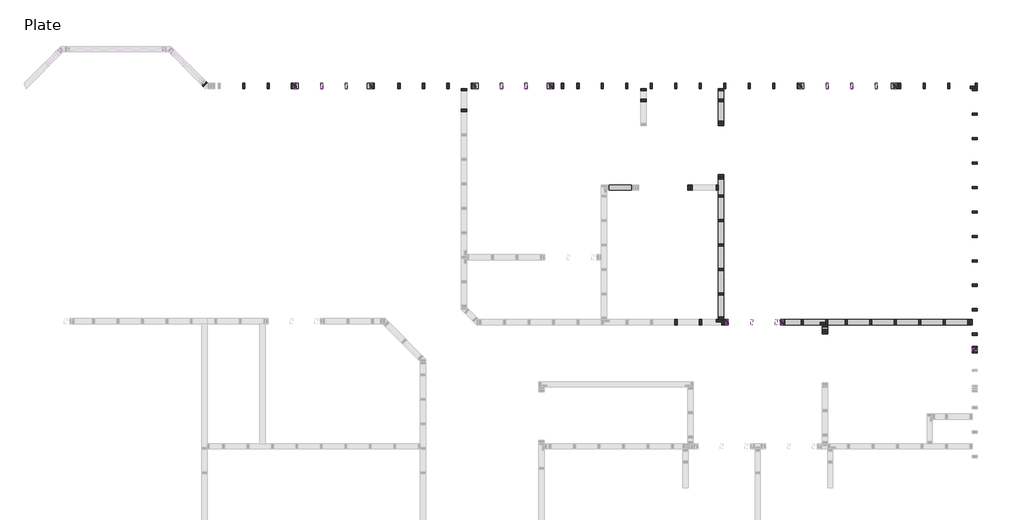
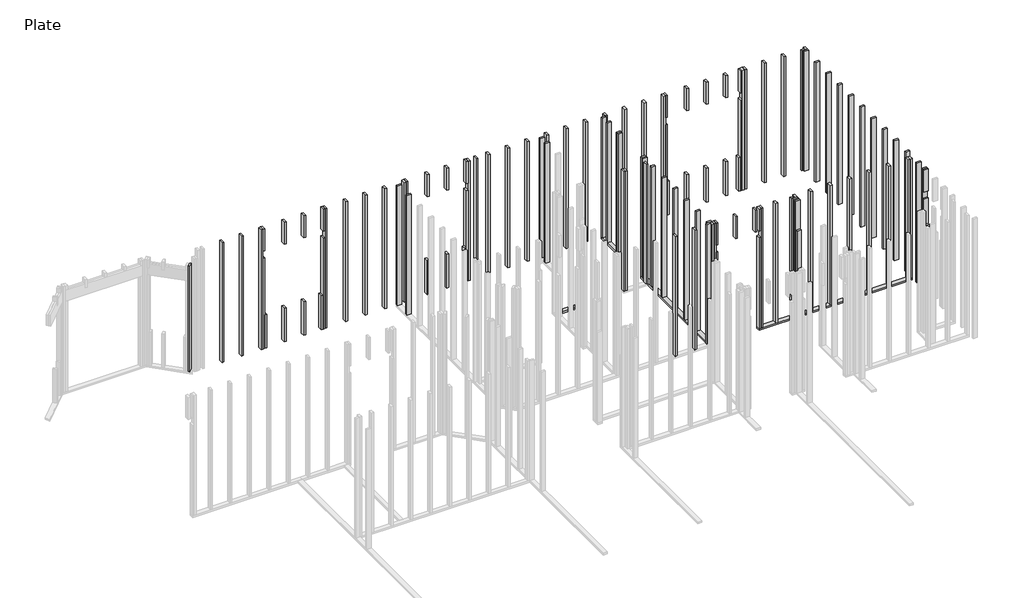
# One storey, part 5 of 5: 118 columns, 5 beams.
# Revit data of these elements (continued)
# Materials (continued)
#   "Softwood, Lumber": class "Wood", colour RGB 223 192 134, transparency 0, Description = "Pinus Echinata", Cost = 0
#   "Douglas Fir #2": class "Wood", colour RGB 223 192 134, transparency 0, Description = "Pinus Echinata", Cost = 0
